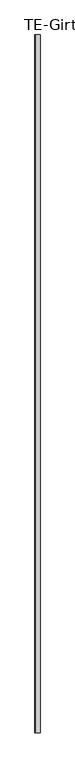
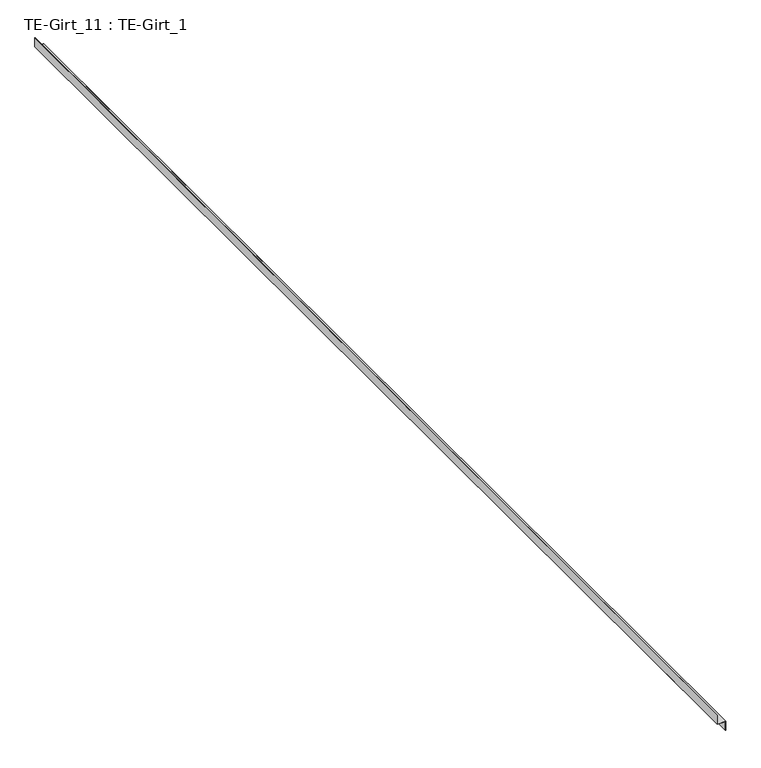
"""IFC4 building model written with IfcOpenShell, lengths in millimetres: proxy geometry, TE-Girt_11 : TE-Girt_1."""

import ifcopenshell
import ifcopenshell.guid

model = None  # the IFC model being written
_history = None  # IfcOwnerHistory: only IFC2X3 demands one
_inside = {}  # id of a spatial element -> (the spatial element, [elements in it])
_under = {}  # id of a project, library or spatial element -> (it, [spatial elements below it])
_declared = {}  # id of a project -> (the project, [libraries it declares])
_typed = {}  # id of a type object -> (the type object, [elements of that type])
_made_of = {}  # id of a material, layer set ... -> (it, [elements and type objects made of it])


def new_model(schema):
    """Start an empty IFC model of exactly this schema.

    Asked for "IFC4X3", IfcOpenShell would pick the latest addendum, in which some entities
    have other attributes; the version numbers below select the first issue.
    IFC2X3 requires an IfcOwnerHistory on every rooted entity: one is made here for all.
    """
    global model, _history
    if schema == "IFC4X3":
        model = ifcopenshell.file(schema_version=(4, 3, 0, 0))
    else:
        model = ifcopenshell.file(schema=schema)
    _inside.clear()
    _under.clear()
    _declared.clear()
    _typed.clear()
    _made_of.clear()
    _history = None
    if model.schema == "IFC2X3":
        org = make("IfcOrganization", Name="unknown")
        user = make(
            "IfcPersonAndOrganization",
            ThePerson=make("IfcPerson", FamilyName="unknown"),
            TheOrganization=org,
        )
        app = make(
            "IfcApplication",
            ApplicationDeveloper=org,
            Version="unknown",
            ApplicationFullName="unknown",
            ApplicationIdentifier="unknown",
        )
        _history = make(
            "IfcOwnerHistory",
            OwningUser=user,
            OwningApplication=app,
            ChangeAction="ADDED",
            CreationDate=0,
        )
    return model


def make(cls, **values):
    """One entity of the class cls with the attributes given. An attribute that is None is left unset."""
    return model.create_entity(
        cls, **{name: value for name, value in values.items() if value is not None}
    )


def rooted(cls, **values):
    """An entity with a GlobalId (a new one), such as an element, a storey or a relation."""
    return make(cls, GlobalId=ifcopenshell.guid.new(), OwnerHistory=_history, **values)


def si_unit(unit_type, name, prefix=None):
    """IfcSIUnit, for example si_unit("LENGTHUNIT", "METRE", prefix="MILLI")."""
    return make("IfcSIUnit", UnitType=unit_type, Prefix=prefix, Name=name)


def assignment(units):
    """IfcUnitAssignment: the units of a project."""
    return None if units is None else make("IfcUnitAssignment", Units=units)


def point(xyz):
    """IfcCartesianPoint."""
    return None if xyz is None else make("IfcCartesianPoint", Coordinates=xyz)


def direction(xyz):
    """IfcDirection."""
    return None if xyz is None else make("IfcDirection", DirectionRatios=xyz)


def frame(location, z_axis=None, x_axis=None):
    """IfcAxis2Placement3D, a coordinate frame: its origin and axes. An axis left out is left unset."""
    return make(
        "IfcAxis2Placement3D",
        Location=point(location),
        Axis=direction(z_axis),
        RefDirection=direction(x_axis),
    )


def origin():
    """The frame at (0, 0, 0) with its axes left unset."""
    return frame((0.0, 0.0, 0.0))


def place(relative_to, where):
    """IfcLocalPlacement: puts the frame where relative to a parent placement (None: the world)."""
    return make(
        "IfcLocalPlacement", PlacementRelTo=relative_to, RelativePlacement=where
    )


def context(
    kind, dimensions, precision=None, world=None, true_north=None, identifier=None
):
    """IfcGeometricRepresentationContext, for example the 3D "Model" context."""
    return make(
        "IfcGeometricRepresentationContext",
        ContextIdentifier=identifier,
        ContextType=kind,
        CoordinateSpaceDimension=dimensions,
        Precision=precision,
        WorldCoordinateSystem=world,
        TrueNorth=true_north,
    )


def project(units=None, contexts=None):
    """IfcProject with its units and contexts."""
    return rooted(
        "IfcProject",
        Name="project",
        RepresentationContexts=contexts,
        UnitsInContext=assignment(units),
    )


def spatial(cls, under=None, at=None, **own):
    """A site, building, storey or space (cls), placed at a placement, below another one or the project."""
    s = rooted(cls, ObjectPlacement=at, **own)
    if under is not None:
        _under.setdefault(under.id(), (under, []))[1].append(s)
    return s


def polyline(points):
    """IfcPolyline through the points."""
    return make("IfcPolyline", Points=[point(p) for p in points])


def outline(outer, holes=None, kind="AREA"):
    """IfcArbitraryClosedProfileDef: a profile drawn as a closed curve; with holes, ...WithVoids."""
    if holes is None:
        return make("IfcArbitraryClosedProfileDef", ProfileType=kind, OuterCurve=outer)
    return make(
        "IfcArbitraryProfileDefWithVoids",
        ProfileType=kind,
        OuterCurve=outer,
        InnerCurves=holes,
    )


def extrude(swept, where, along, depth):
    """IfcExtrudedAreaSolid: the profile swept, set in the frame where, extruded along a direction by depth."""
    return make(
        "IfcExtrudedAreaSolid",
        SweptArea=swept,
        Position=where,
        ExtrudedDirection=direction(along),
        Depth=depth,
    )


def shape(context_of_items, identifier, shape_type, items):
    """IfcShapeRepresentation: the items that make up one representation, for example the "Body"."""
    return make(
        "IfcShapeRepresentation",
        ContextOfItems=context_of_items,
        RepresentationIdentifier=identifier,
        RepresentationType=shape_type,
        Items=items,
    )


def source(mapping_origin, context_of_items, identifier, shape_type, items):
    """IfcRepresentationMap: a shape defined once, which mapped items show again and again."""
    return make(
        "IfcRepresentationMap",
        MappingOrigin=mapping_origin,
        MappedRepresentation=shape(context_of_items, identifier, shape_type, items),
    )


def transform(
    local_origin,
    x_axis=None,
    y_axis=None,
    z_axis=None,
    scale=None,
    scale2=None,
    scale3=None,
    uniform=True,
):
    """IfcCartesianTransformationOperator3D, or its non-uniform kind. x_axis, y_axis, z_axis: its Axis1, 2, 3."""
    if uniform:
        return make(
            "IfcCartesianTransformationOperator3D",
            Axis1=direction(x_axis),
            Axis2=direction(y_axis),
            LocalOrigin=point(local_origin),
            Scale=scale,
            Axis3=direction(z_axis),
        )
    return make(
        "IfcCartesianTransformationOperator3DnonUniform",
        Axis1=direction(x_axis),
        Axis2=direction(y_axis),
        LocalOrigin=point(local_origin),
        Scale=scale,
        Axis3=direction(z_axis),
        Scale2=scale2,
        Scale3=scale3,
    )


def mapped(mapping_source, mapping_target):
    """IfcMappedItem: shows the shape of a source again, moved by a transform."""
    return make(
        "IfcMappedItem", MappingSource=mapping_source, MappingTarget=mapping_target
    )


def made_of(thing, what):
    """Note that an element or type object is made of a material, layer set ...; save() writes the relation."""
    if what is not None:
        _made_of.setdefault(what.id(), (what, []))[1].append(thing)
    return thing


def element(
    cls,
    number,
    at=None,
    inside=None,
    cuts=None,
    type_object=None,
    material=None,
    context=None,
    identifier="Body",
    shape_type=None,
    held_by="IfcProductDefinitionShape",
    body=None,
    shapes=None,
    **own,
):
    """One element of the class cls, such as IfcWall. Its Tag is "e" and its number.

    at: its placement. inside: the storey or other place that contains it. cuts: it is an
    opening in that element (IfcRelVoidsElement). A single representation is given by context,
    identifier, shape_type and body (its items); several are given by shapes. held_by: the class
    of the entity that holds the representations. save() writes the other relations.
    """
    e = rooted(cls, Tag="e%d" % number, ObjectPlacement=at, **own)
    if body is not None:
        shapes = [shape(context, identifier, shape_type, body)]
    if shapes is not None:
        e.Representation = make(held_by, Representations=shapes)
    if inside is not None:
        _inside.setdefault(inside.id(), (inside, []))[1].append(e)
    if cuts is not None:
        rooted(
            "IfcRelVoidsElement", RelatingBuildingElement=cuts, RelatedOpeningElement=e
        )
    if type_object is not None:
        _typed.setdefault(type_object.id(), (type_object, []))[1].append(e)
    return made_of(e, material)


def aggregate(whole, parts):
    """IfcRelAggregates: a whole, such as a stair, and the parts it consists of."""
    return rooted("IfcRelAggregates", RelatingObject=whole, RelatedObjects=parts)


def save(model, path):
    """Write the relations noted so far, then the file.

    IfcRelAggregates (storeys below a building ...), IfcRelContainedInSpatialStructure (elements
    in a storey), IfcRelDefinesByType, IfcRelAssociatesMaterial and IfcRelDeclares: one each for
    every whole, place, type object, material and project.
    """
    for whole, parts in _under.values():
        aggregate(whole, parts)
    for where, things in _inside.values():
        rooted(
            "IfcRelContainedInSpatialStructure",
            RelatedElements=things,
            RelatingStructure=where,
        )
    for kind, things in _typed.values():
        rooted("IfcRelDefinesByType", RelatedObjects=things, RelatingType=kind)
    for what, things in _made_of.values():
        rooted("IfcRelAssociatesMaterial", RelatedObjects=things, RelatingMaterial=what)
    for by, libraries in _declared.values():
        rooted("IfcRelDeclares", RelatingContext=by, RelatedDefinitions=libraries)
    model.write(path)


def te_girt_11_te_girt_1_7c41e33f(model_context):
    return source(origin(), model_context, "Body", "SweptSolid", [
        extrude(outline(polyline([(1657.35, 590353.5520246), (1657.35, 590319.5364427), (1694.5570313, 590319.5364427), (1694.5570313, 590318.6434739), (1656.4570313, 590318.6434739), (1656.4570313, 590352.6590559), (1619.25, 590352.6590559), (1619.25, 590353.5520246), (1657.35, 590353.5520246)])), frame((0.0, -536417.5913841, 0.0), z_axis=(0.0, 1.0, 0.0), x_axis=(0.0, 0.0, 1.0)), (0.0, 0.0, 1.0), 4778.375),
    ])


if __name__ == "__main__":
    model = new_model("IFC4")
    model_context = context("Model", 3, world=origin())
    ifc_project = project(units=[si_unit("LENGTHUNIT", "METRE", prefix="MILLI")], contexts=[model_context])
    site = spatial("IfcSite", under=ifc_project)
    building = spatial("IfcBuilding", under=site)
    placement = place(None, origin())
    te_girt_11_te_girt_1_shape = te_girt_11_te_girt_1_7c41e33f(model_context)
    element("IfcBuildingElementProxy", 1, Name="TE-Girt_11 : TE-Girt_1", ObjectType="TE-Girt_11 : TE-Girt_1", at=placement, inside=building, context=model_context, shape_type="MappedRepresentation", body=[
        mapped(te_girt_11_te_girt_1_shape, transform((0.0, 0.0, 0.0), x_axis=(1.0, 0.0, 0.0), y_axis=(0.0, 1.0, 0.0), z_axis=(0.0, 0.0, 1.0))),
    ])
    save(model, "model.ifc")

# Revit data of these elements
# Element 1 (IfcBuildingElementProxy, "TE-Girt_11 : TE-Girt_1")
#   Materials on its faces: "Z-FURRING, COLD-FORMED GALV."
# Materials
#   "Z-FURRING, COLD-FORMED GALV.": class "Generic", colour RGB 143 142 141, transparency 0, Cost = 0
